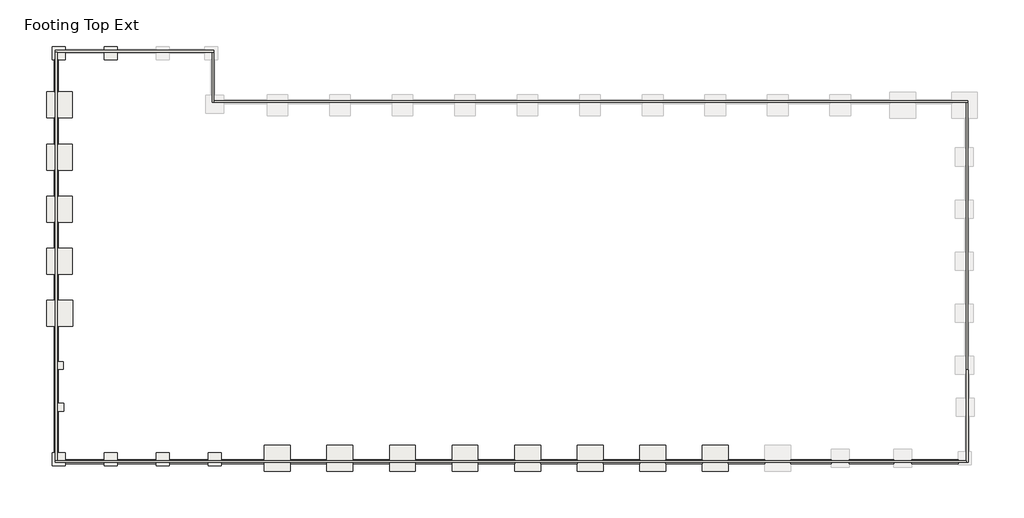
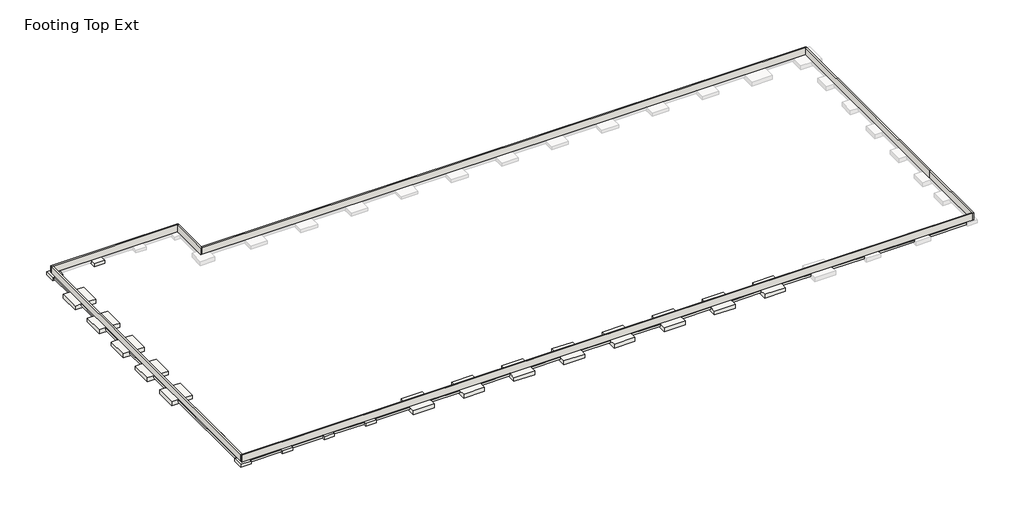
# One storey, part 1 of 2: 21 slabs, 7 walls, 2 footings.
"""IFC4 building model written with IfcOpenShell, lengths in millimetres."""

from ifc_helpers import new_model, si_unit, frame, origin, place, context, project, spatial, polyline, outline, extrude, faceted_brep, element, save

model = new_model("IFC4")

# Units and contexts
model_context = context("Model", 3, world=origin())
ifc_project = project(units=[si_unit("LENGTHUNIT", "METRE", prefix="MILLI")], contexts=[model_context])

# Site, building, storey
site = spatial("IfcSite", under=ifc_project)
building = spatial("IfcBuilding", under=site)
storey = spatial("IfcBuildingStorey", under=building, Name="Footing Top Ext", Elevation=-1066.8)

# Footings
placement = place(None, origin())
element("IfcFooting", 1, ObjectType="Bearing Footing - 18\" x 12\"", at=placement, inside=storey, context=model_context, shape_type="SweptSolid", body=[
    extrude(outline(polyline([(305655.7648264, -579216.5913841), (305655.7648264, -578759.3913841), (310230.9398264, -578759.3913841), (310230.9398264, -579216.5913841), (305655.7648264, -579216.5913841)])), frame((0.0, 0.0, -1371.6), z_axis=(0.0, 0.0, 1.0), x_axis=(1.0, 0.0, 0.0)), (0.0, 0.0, 1.0), 304.8),
    extrude(outline(polyline([(311754.9398264, -579216.5913841), (311754.9398264, -578759.3913841), (316361.8648264, -578759.3913841), (316361.8648264, -579216.5913841), (311754.9398264, -579216.5913841)])), frame((0.0, 0.0, -1371.6), z_axis=(0.0, 0.0, 1.0), x_axis=(1.0, 0.0, 0.0)), (0.0, 0.0, 1.0), 304.8),
    extrude(outline(polyline([(317885.8648264, -579216.5913841), (317885.8648264, -578759.3913841), (322457.8648264, -578759.3913841), (322457.8648264, -579216.5913841), (317885.8648264, -579216.5913841)])), frame((0.0, 0.0, -1371.6), z_axis=(0.0, 0.0, 1.0), x_axis=(1.0, 0.0, 0.0)), (0.0, 0.0, 1.0), 304.8),
    extrude(outline(polyline([(323981.8648264, -579216.5913841), (323981.8648264, -578759.3913841), (329077.7398264, -578759.3913841), (329077.7398264, -579216.5913841), (323981.8648264, -579216.5913841)])), frame((0.0, 0.0, -1371.6), z_axis=(0.0, 0.0, 1.0), x_axis=(1.0, 0.0, 0.0)), (0.0, 0.0, 1.0), 304.8),
    extrude(outline(polyline([(332125.7398264, -579216.5913841), (332125.7398264, -578759.3913841), (336431.0398264, -578759.3913841), (336431.0398264, -579216.5913841), (332125.7398264, -579216.5913841)])), frame((0.0, 0.0, -1371.6), z_axis=(0.0, 0.0, 1.0), x_axis=(1.0, 0.0, 0.0)), (0.0, 0.0, 1.0), 304.8),
    extrude(outline(polyline([(339479.0398264, -579216.5913841), (339479.0398264, -578759.3913841), (343784.3398264, -578759.3913841), (343784.3398264, -579216.5913841), (339479.0398264, -579216.5913841)])), frame((0.0, 0.0, -1371.6), z_axis=(0.0, 0.0, 1.0), x_axis=(1.0, 0.0, 0.0)), (0.0, 0.0, 1.0), 304.8),
    extrude(outline(polyline([(346832.3398264, -579216.5913841), (346832.3398264, -578759.3913841), (351137.6398264, -578759.3913841), (351137.6398264, -579216.5913841), (346832.3398264, -579216.5913841)])), frame((0.0, 0.0, -1371.6), z_axis=(0.0, 0.0, 1.0), x_axis=(1.0, 0.0, 0.0)), (0.0, 0.0, 1.0), 304.8),
    extrude(outline(polyline([(354185.6398264, -579216.5913841), (354185.6398264, -578759.3913841), (358490.9398264, -578759.3913841), (358490.9398264, -579216.5913841), (354185.6398264, -579216.5913841)])), frame((0.0, 0.0, -1371.6), z_axis=(0.0, 0.0, 1.0), x_axis=(1.0, 0.0, 0.0)), (0.0, 0.0, 1.0), 304.8),
    extrude(outline(polyline([(361538.9398264, -579216.5913841), (361538.9398264, -578759.3913841), (365844.2398264, -578759.3913841), (365844.2398264, -579216.5913841), (361538.9398264, -579216.5913841)])), frame((0.0, 0.0, -1371.6), z_axis=(0.0, 0.0, 1.0), x_axis=(1.0, 0.0, 0.0)), (0.0, 0.0, 1.0), 304.8),
    extrude(outline(polyline([(368892.2398264, -579216.5913841), (368892.2398264, -578759.3913841), (373197.5398264, -578759.3913841), (373197.5398264, -579216.5913841), (368892.2398264, -579216.5913841)])), frame((0.0, 0.0, -1371.6), z_axis=(0.0, 0.0, 1.0), x_axis=(1.0, 0.0, 0.0)), (0.0, 0.0, 1.0), 304.8),
    extrude(outline(polyline([(376245.5398264, -579216.5913841), (376245.5398264, -578759.3913841), (380550.8398264, -578759.3913841), (380550.8398264, -579216.5913841), (376245.5398264, -579216.5913841)])), frame((0.0, 0.0, -1371.6), z_axis=(0.0, 0.0, 1.0), x_axis=(1.0, 0.0, 0.0)), (0.0, 0.0, 1.0), 304.8),
    extrude(outline(polyline([(383598.8398264, -579216.5913841), (383598.8398264, -578759.3913841), (387904.1398264, -578759.3913841), (387904.1398264, -579216.5913841), (383598.8398264, -579216.5913841)])), frame((0.0, 0.0, -1371.6), z_axis=(0.0, 0.0, 1.0), x_axis=(1.0, 0.0, 0.0)), (0.0, 0.0, 1.0), 304.8),
    extrude(outline(polyline([(390952.1398264, -579216.5913841), (390952.1398264, -578759.3913841), (395714.6398264, -578759.3913841), (395714.6398264, -579216.5913841), (390952.1398264, -579216.5913841)])), frame((0.0, 0.0, -1371.6), z_axis=(0.0, 0.0, 1.0), x_axis=(1.0, 0.0, 0.0)), (0.0, 0.0, 1.0), 304.8),
    extrude(outline(polyline([(397848.2398264, -579216.5913841), (397848.2398264, -578759.3913841), (403067.9398264, -578759.3913841), (403067.9398264, -579216.5913841), (397848.2398264, -579216.5913841)])), frame((0.0, 0.0, -1371.6), z_axis=(0.0, 0.0, 1.0), x_axis=(1.0, 0.0, 0.0)), (0.0, 0.0, 1.0), 304.8),
    extrude(outline(polyline([(405201.5398264, -579216.5913841), (405201.5398264, -578759.3913841), (410675.2398264, -578759.3913841), (410675.2398264, -579216.5913841), (405201.5398264, -579216.5913841)])), frame((0.0, 0.0, -1371.6), z_axis=(0.0, 0.0, 1.0), x_axis=(1.0, 0.0, 0.0)), (0.0, 0.0, 1.0), 304.8),
])
element("IfcFooting", 2, ObjectType="Bearing Footing - 18\" x 12\"", at=placement, inside=storey, context=model_context, shape_type="SweptSolid", body=[
    extrude(outline(polyline([(304369.8898264, -531712.2413841), (304827.0898264, -531712.2413841), (304827.0898264, -535528.5913841), (304369.8898264, -535528.5913841), (304369.8898264, -531712.2413841)])), frame((0.0, 0.0, -1371.6), z_axis=(0.0, 0.0, 1.0), x_axis=(1.0, 0.0, 0.0)), (0.0, 0.0, 1.0), 304.8),
    extrude(outline(polyline([(304369.8898264, -538576.5913841), (304827.0898264, -538576.5913841), (304827.0898264, -541656.3413841), (304369.8898264, -541656.3413841), (304369.8898264, -538576.5913841)])), frame((0.0, 0.0, -1371.6), z_axis=(0.0, 0.0, 1.0), x_axis=(1.0, 0.0, 0.0)), (0.0, 0.0, 1.0), 304.8),
    extrude(outline(polyline([(304369.8898264, -544704.3413841), (304827.0898264, -544704.3413841), (304827.0898264, -547784.0913841), (304369.8898264, -547784.0913841), (304369.8898264, -544704.3413841)])), frame((0.0, 0.0, -1371.6), z_axis=(0.0, 0.0, 1.0), x_axis=(1.0, 0.0, 0.0)), (0.0, 0.0, 1.0), 304.8),
    extrude(outline(polyline([(304369.8898264, -550832.0913841), (304827.0898264, -550832.0913841), (304827.0898264, -553911.8413841), (304369.8898264, -553911.8413841), (304369.8898264, -550832.0913841)])), frame((0.0, 0.0, -1371.6), z_axis=(0.0, 0.0, 1.0), x_axis=(1.0, 0.0, 0.0)), (0.0, 0.0, 1.0), 304.8),
    extrude(outline(polyline([(304369.8898264, -556959.8413841), (304827.0898264, -556959.8413841), (304827.0898264, -560039.5913841), (304369.8898264, -560039.5913841), (304369.8898264, -556959.8413841)])), frame((0.0, 0.0, -1371.6), z_axis=(0.0, 0.0, 1.0), x_axis=(1.0, 0.0, 0.0)), (0.0, 0.0, 1.0), 304.8),
    extrude(outline(polyline([(304369.8898264, -563087.5913841), (304827.0898264, -563087.5913841), (304827.0898264, -567234.1413841), (304528.6398264, -567234.1413841), (304528.6398264, -568148.5413841), (304827.0898264, -568148.5413841), (304827.0898264, -572136.3413841), (304585.7898264, -572136.3413841), (304585.7898264, -573050.7413841), (304827.0898264, -573050.7413841), (304827.0898264, -577933.8913841), (304369.8898264, -577933.8913841), (304369.8898264, -563087.5913841)])), frame((0.0, 0.0, -1371.6), z_axis=(0.0, 0.0, 1.0), x_axis=(1.0, 0.0, 0.0)), (0.0, 0.0, 1.0), 304.8),
])

# Slabs
element("IfcSlab", 3, ObjectType="Footing-Rectangular : F10", at=placement, inside=storey, context=model_context, shape_type="Brep", body=[
    faceted_brep([(306509.8398264, -535528.5913841, -1066.8), (304827.0898264, -535528.5913841, -1066.8), (304369.8898264, -535528.5913841, -1066.8), (303461.8398264, -535528.5913841, -1066.8), (303461.8398264, -538576.5913841, -1066.8), (304369.8898264, -538576.5913841, -1066.8), (304827.0898264, -538576.5913841, -1066.8), (306509.8398264, -538576.5913841, -1066.8), (306509.8398264, -535528.5913841, -1676.4), (306509.8398264, -538576.5913841, -1676.4), (303461.8398264, -538576.5913841, -1676.4), (303461.8398264, -535528.5913841, -1676.4)], [[[0, 1, 2, 3, 4, 5, 6, 7]], [[8, 9, 10, 11]], [[3, 2, 1, 0, 8, 11]], [[4, 3, 11, 10]], [[7, 6, 5, 4, 10, 9]], [[0, 7, 9, 8]]]),
])
element("IfcSlab", 4, ObjectType="Footing-Rectangular : F10", at=placement, inside=storey, context=model_context, shape_type="Brep", body=[
    faceted_brep([(306509.8398264, -541656.3413841, -1066.8), (304827.0898264, -541656.3413841, -1066.8), (304369.8898264, -541656.3413841, -1066.8), (303461.8398264, -541656.3413841, -1066.8), (303461.8398264, -544704.3413841, -1066.8), (304369.8898264, -544704.3413841, -1066.8), (304827.0898264, -544704.3413841, -1066.8), (306509.8398264, -544704.3413841, -1066.8), (306509.8398264, -541656.3413841, -1676.4), (306509.8398264, -544704.3413841, -1676.4), (303461.8398264, -544704.3413841, -1676.4), (303461.8398264, -541656.3413841, -1676.4)], [[[0, 1, 2, 3, 4, 5, 6, 7]], [[8, 9, 10, 11]], [[3, 2, 1, 0, 8, 11]], [[4, 3, 11, 10]], [[7, 6, 5, 4, 10, 9]], [[0, 7, 9, 8]]]),
])
element("IfcSlab", 5, ObjectType="Footing-Rectangular : F10", at=placement, inside=storey, context=model_context, shape_type="Brep", body=[
    faceted_brep([(306509.8398264, -547784.0913841, -1066.8), (304827.0898264, -547784.0913841, -1066.8), (304369.8898264, -547784.0913841, -1066.8), (303461.8398264, -547784.0913841, -1066.8), (303461.8398264, -550832.0913841, -1066.8), (304369.8898264, -550832.0913841, -1066.8), (304827.0898264, -550832.0913841, -1066.8), (306509.8398264, -550832.0913841, -1066.8), (306509.8398264, -547784.0913841, -1676.4), (306509.8398264, -550832.0913841, -1676.4), (303461.8398264, -550832.0913841, -1676.4), (303461.8398264, -547784.0913841, -1676.4)], [[[0, 1, 2, 3, 4, 5, 6, 7]], [[8, 9, 10, 11]], [[3, 2, 1, 0, 8, 11]], [[4, 3, 11, 10]], [[7, 6, 5, 4, 10, 9]], [[0, 7, 9, 8]]]),
])
element("IfcSlab", 6, ObjectType="Footing-Rectangular : F10", at=placement, inside=storey, context=model_context, shape_type="Brep", body=[
    faceted_brep([(306509.8398264, -553911.8413841, -1066.8), (304827.0898264, -553911.8413841, -1066.8), (304369.8898264, -553911.8413841, -1066.8), (303461.8398264, -553911.8413841, -1066.8), (303461.8398264, -556959.8413841, -1066.8), (304369.8898264, -556959.8413841, -1066.8), (304827.0898264, -556959.8413841, -1066.8), (306509.8398264, -556959.8413841, -1066.8), (306509.8398264, -553911.8413841, -1676.4), (306509.8398264, -556959.8413841, -1676.4), (303461.8398264, -556959.8413841, -1676.4), (303461.8398264, -553911.8413841, -1676.4)], [[[0, 1, 2, 3, 4, 5, 6, 7]], [[8, 9, 10, 11]], [[3, 2, 1, 0, 8, 11]], [[4, 3, 11, 10]], [[7, 6, 5, 4, 10, 9]], [[0, 7, 9, 8]]]),
])
element("IfcSlab", 7, ObjectType="Footing-Rectangular : F10", at=placement, inside=storey, context=model_context, shape_type="Brep", body=[
    faceted_brep([(306516.1898264, -560039.5913841, -1066.8), (304827.0898264, -560039.5913841, -1066.8), (304369.8898264, -560039.5913841, -1066.8), (303468.1898264, -560039.5913841, -1066.8), (303468.1898264, -563087.5913841, -1066.8), (304369.8898264, -563087.5913841, -1066.8), (304827.0898264, -563087.5913841, -1066.8), (306516.1898264, -563087.5913841, -1066.8), (306516.1898264, -560039.5913841, -1676.4), (306516.1898264, -563087.5913841, -1676.4), (303468.1898264, -563087.5913841, -1676.4), (303468.1898264, -560039.5913841, -1676.4)], [[[0, 1, 2, 3, 4, 5, 6, 7]], [[8, 9, 10, 11]], [[3, 2, 1, 0, 8, 11]], [[4, 3, 11, 10]], [[7, 6, 5, 4, 10, 9]], [[0, 7, 9, 8]]]),
])
element("IfcSlab", 8, ObjectType="Footing-Rectangular : F10", at=placement, inside=storey, context=model_context, shape_type="Brep", body=[
    faceted_brep([(332125.7398264, -577079.8163841, -1066.8), (329077.7398264, -577079.8163841, -1066.8), (329077.7398264, -578759.3913841, -1066.8), (329077.7398264, -579216.5913841, -1066.8), (329077.7398264, -580127.8163841, -1066.8), (332125.7398264, -580127.8163841, -1066.8), (332125.7398264, -579216.5913841, -1066.8), (332125.7398264, -578759.3913841, -1066.8), (332125.7398264, -577079.8163841, -1676.4), (332125.7398264, -580127.8163841, -1676.4), (329077.7398264, -580127.8163841, -1676.4), (329077.7398264, -577079.8163841, -1676.4)], [[[0, 1, 2, 3, 4, 5, 6, 7]], [[8, 9, 10, 11]], [[1, 0, 8, 11]], [[4, 3, 2, 1, 11, 10]], [[5, 4, 10, 9]], [[0, 7, 6, 5, 9, 8]]]),
])
element("IfcSlab", 9, ObjectType="Footing-Rectangular : F10", at=placement, inside=storey, context=model_context, shape_type="Brep", body=[
    faceted_brep([(339479.0398264, -577079.8163841, -1066.8), (336431.0398264, -577079.8163841, -1066.8), (336431.0398264, -578759.3913841, -1066.8), (336431.0398264, -579216.5913841, -1066.8), (336431.0398264, -580127.8163841, -1066.8), (339479.0398264, -580127.8163841, -1066.8), (339479.0398264, -579216.5913841, -1066.8), (339479.0398264, -578759.3913841, -1066.8), (339479.0398264, -577079.8163841, -1676.4), (339479.0398264, -580127.8163841, -1676.4), (336431.0398264, -580127.8163841, -1676.4), (336431.0398264, -577079.8163841, -1676.4)], [[[0, 1, 2, 3, 4, 5, 6, 7]], [[8, 9, 10, 11]], [[1, 0, 8, 11]], [[4, 3, 2, 1, 11, 10]], [[5, 4, 10, 9]], [[0, 7, 6, 5, 9, 8]]]),
])
element("IfcSlab", 10, ObjectType="Footing-Rectangular : F10", at=placement, inside=storey, context=model_context, shape_type="Brep", body=[
    faceted_brep([(346832.3398264, -577079.8163841, -1066.8), (343784.3398264, -577079.8163841, -1066.8), (343784.3398264, -578759.3913841, -1066.8), (343784.3398264, -579216.5913841, -1066.8), (343784.3398264, -580127.8163841, -1066.8), (346832.3398264, -580127.8163841, -1066.8), (346832.3398264, -579216.5913841, -1066.8), (346832.3398264, -578759.3913841, -1066.8), (346832.3398264, -577079.8163841, -1676.4), (346832.3398264, -580127.8163841, -1676.4), (343784.3398264, -580127.8163841, -1676.4), (343784.3398264, -577079.8163841, -1676.4)], [[[0, 1, 2, 3, 4, 5, 6, 7]], [[8, 9, 10, 11]], [[1, 0, 8, 11]], [[4, 3, 2, 1, 11, 10]], [[5, 4, 10, 9]], [[0, 7, 6, 5, 9, 8]]]),
])
element("IfcSlab", 11, ObjectType="Footing-Rectangular : F10", at=placement, inside=storey, context=model_context, shape_type="Brep", body=[
    faceted_brep([(354185.6398264, -577079.8163841, -1066.8), (351137.6398264, -577079.8163841, -1066.8), (351137.6398264, -578759.3913841, -1066.8), (351137.6398264, -579216.5913841, -1066.8), (351137.6398264, -580127.8163841, -1066.8), (354185.6398264, -580127.8163841, -1066.8), (354185.6398264, -579216.5913841, -1066.8), (354185.6398264, -578759.3913841, -1066.8), (354185.6398264, -577079.8163841, -1676.4), (354185.6398264, -580127.8163841, -1676.4), (351137.6398264, -580127.8163841, -1676.4), (351137.6398264, -577079.8163841, -1676.4)], [[[0, 1, 2, 3, 4, 5, 6, 7]], [[8, 9, 10, 11]], [[1, 0, 8, 11]], [[4, 3, 2, 1, 11, 10]], [[5, 4, 10, 9]], [[0, 7, 6, 5, 9, 8]]]),
])
element("IfcSlab", 12, ObjectType="Footing-Rectangular : F10", at=placement, inside=storey, context=model_context, shape_type="Brep", body=[
    faceted_brep([(361538.9398264, -577079.8163841, -1066.8), (358490.9398264, -577079.8163841, -1066.8), (358490.9398264, -578759.3913841, -1066.8), (358490.9398264, -579216.5913841, -1066.8), (358490.9398264, -580127.8163841, -1066.8), (361538.9398264, -580127.8163841, -1066.8), (361538.9398264, -579216.5913841, -1066.8), (361538.9398264, -578759.3913841, -1066.8), (361538.9398264, -577079.8163841, -1676.4), (361538.9398264, -580127.8163841, -1676.4), (358490.9398264, -580127.8163841, -1676.4), (358490.9398264, -577079.8163841, -1676.4)], [[[0, 1, 2, 3, 4, 5, 6, 7]], [[8, 9, 10, 11]], [[1, 0, 8, 11]], [[4, 3, 2, 1, 11, 10]], [[5, 4, 10, 9]], [[0, 7, 6, 5, 9, 8]]]),
])
element("IfcSlab", 13, ObjectType="Footing-Rectangular : F10", at=placement, inside=storey, context=model_context, shape_type="Brep", body=[
    faceted_brep([(368892.2398264, -577079.8163841, -1066.8), (365844.2398264, -577079.8163841, -1066.8), (365844.2398264, -578759.3913841, -1066.8), (365844.2398264, -579216.5913841, -1066.8), (365844.2398264, -580127.8163841, -1066.8), (368892.2398264, -580127.8163841, -1066.8), (368892.2398264, -579216.5913841, -1066.8), (368892.2398264, -578759.3913841, -1066.8), (368892.2398264, -577079.8163841, -1676.4), (368892.2398264, -580127.8163841, -1676.4), (365844.2398264, -580127.8163841, -1676.4), (365844.2398264, -577079.8163841, -1676.4)], [[[0, 1, 2, 3, 4, 5, 6, 7]], [[8, 9, 10, 11]], [[1, 0, 8, 11]], [[4, 3, 2, 1, 11, 10]], [[5, 4, 10, 9]], [[0, 7, 6, 5, 9, 8]]]),
])
element("IfcSlab", 14, ObjectType="Footing-Rectangular : F10", at=placement, inside=storey, context=model_context, shape_type="Brep", body=[
    faceted_brep([(376245.5398264, -577079.8163841, -1066.8), (373197.5398264, -577079.8163841, -1066.8), (373197.5398264, -578759.3913841, -1066.8), (373197.5398264, -579216.5913841, -1066.8), (373197.5398264, -580127.8163841, -1066.8), (376245.5398264, -580127.8163841, -1066.8), (376245.5398264, -579216.5913841, -1066.8), (376245.5398264, -578759.3913841, -1066.8), (376245.5398264, -577079.8163841, -1676.4), (376245.5398264, -580127.8163841, -1676.4), (373197.5398264, -580127.8163841, -1676.4), (373197.5398264, -577079.8163841, -1676.4)], [[[0, 1, 2, 3, 4, 5, 6, 7]], [[8, 9, 10, 11]], [[1, 0, 8, 11]], [[4, 3, 2, 1, 11, 10]], [[5, 4, 10, 9]], [[0, 7, 6, 5, 9, 8]]]),
])
element("IfcSlab", 15, ObjectType="Footing-Rectangular : F10", at=placement, inside=storey, context=model_context, shape_type="Brep", body=[
    faceted_brep([(383598.8398264, -577079.8163841, -1066.8), (380550.8398264, -577079.8163841, -1066.8), (380550.8398264, -578759.3913841, -1066.8), (380550.8398264, -579216.5913841, -1066.8), (380550.8398264, -580127.8163841, -1066.8), (383598.8398264, -580127.8163841, -1066.8), (383598.8398264, -579216.5913841, -1066.8), (383598.8398264, -578759.3913841, -1066.8), (383598.8398264, -577079.8163841, -1676.4), (383598.8398264, -580127.8163841, -1676.4), (380550.8398264, -580127.8163841, -1676.4), (380550.8398264, -577079.8163841, -1676.4)], [[[0, 1, 2, 3, 4, 5, 6, 7]], [[8, 9, 10, 11]], [[1, 0, 8, 11]], [[4, 3, 2, 1, 11, 10]], [[5, 4, 10, 9]], [[0, 7, 6, 5, 9, 8]]]),
])
element("IfcSlab", 16, ObjectType="Footing-Rectangular : F5", at=placement, inside=storey, context=model_context, shape_type="Brep", body=[
    faceted_brep([(305655.7648264, -530188.2413841, -1066.8), (304131.7648264, -530188.2413841, -1066.8), (304131.7648264, -531712.2413841, -1066.8), (304369.8898264, -531712.2413841, -1066.8), (304827.0898264, -531712.2413841, -1066.8), (305655.7648264, -531712.2413841, -1066.8), (305655.7648264, -530975.6413841, -1066.8), (305655.7648264, -530518.4413841, -1066.8), (305655.7648264, -530188.2413841, -1524.0), (305655.7648264, -531712.2413841, -1524.0), (304131.7648264, -531712.2413841, -1524.0), (304131.7648264, -530188.2413841, -1524.0)], [[[0, 1, 2, 3, 4, 5, 6, 7]], [[8, 9, 10, 11]], [[1, 0, 8, 11]], [[2, 1, 11, 10]], [[5, 4, 3, 2, 10, 9]], [[0, 7, 6, 5, 9, 8]]]),
])
element("IfcSlab", 17, ObjectType="Footing-Rectangular : F5", at=placement, inside=storey, context=model_context, shape_type="Brep", body=[
    faceted_brep([(311754.9398264, -530191.4163841, -1066.8), (310230.9398264, -530191.4163841, -1066.8), (310230.9398264, -530518.4413841, -1066.8), (310230.9398264, -530975.6413841, -1066.8), (310230.9398264, -531715.4163841, -1066.8), (311754.9398264, -531715.4163841, -1066.8), (311754.9398264, -530975.6413841, -1066.8), (311754.9398264, -530518.4413841, -1066.8), (311754.9398264, -530191.4163841, -1524.0), (311754.9398264, -531715.4163841, -1524.0), (310230.9398264, -531715.4163841, -1524.0), (310230.9398264, -530191.4163841, -1524.0)], [[[0, 1, 2, 3, 4, 5, 6, 7]], [[8, 9, 10, 11]], [[1, 0, 8, 11]], [[4, 3, 2, 1, 11, 10]], [[5, 4, 10, 9]], [[0, 7, 6, 5, 9, 8]]]),
])
element("IfcSlab", 18, ObjectType="Footing-Rectangular : F5", at=placement, inside=storey, context=model_context, shape_type="Brep", body=[
    faceted_brep([(305655.7648264, -577933.8913841, -1066.8), (304827.0898264, -577933.8913841, -1066.8), (304369.8898264, -577933.8913841, -1066.8), (304131.7648264, -577933.8913841, -1066.8), (304131.7648264, -579457.8913841, -1066.8), (305655.7648264, -579457.8913841, -1066.8), (305655.7648264, -579216.5913841, -1066.8), (305655.7648264, -578759.3913841, -1066.8), (305655.7648264, -577933.8913841, -1524.0), (305655.7648264, -579457.8913841, -1524.0), (304131.7648264, -579457.8913841, -1524.0), (304131.7648264, -577933.8913841, -1524.0)], [[[0, 1, 2, 3, 4, 5, 6, 7]], [[8, 9, 10, 11]], [[3, 2, 1, 0, 8, 11]], [[4, 3, 11, 10]], [[5, 4, 10, 9]], [[0, 7, 6, 5, 9, 8]]]),
])
element("IfcSlab", 19, ObjectType="Footing-Rectangular : F5", at=placement, inside=storey, context=model_context, shape_type="Brep", body=[
    faceted_brep([(311754.9398264, -577930.7163841, -1066.8), (310230.9398264, -577930.7163841, -1066.8), (310230.9398264, -578759.3913841, -1066.8), (310230.9398264, -579216.5913841, -1066.8), (310230.9398264, -579454.7163841, -1066.8), (311754.9398264, -579454.7163841, -1066.8), (311754.9398264, -579216.5913841, -1066.8), (311754.9398264, -578759.3913841, -1066.8), (311754.9398264, -577930.7163841, -1524.0), (311754.9398264, -579454.7163841, -1524.0), (310230.9398264, -579454.7163841, -1524.0), (310230.9398264, -577930.7163841, -1524.0)], [[[0, 1, 2, 3, 4, 5, 6, 7]], [[8, 9, 10, 11]], [[1, 0, 8, 11]], [[4, 3, 2, 1, 11, 10]], [[5, 4, 10, 9]], [[0, 7, 6, 5, 9, 8]]]),
])
element("IfcSlab", 20, ObjectType="Footing-Rectangular : F5", at=placement, inside=storey, context=model_context, shape_type="Brep", body=[
    faceted_brep([(317885.8648264, -577930.7163841, -1066.8), (316361.8648264, -577930.7163841, -1066.8), (316361.8648264, -578759.3913841, -1066.8), (316361.8648264, -579216.5913841, -1066.8), (316361.8648264, -579454.7163841, -1066.8), (317885.8648264, -579454.7163841, -1066.8), (317885.8648264, -579216.5913841, -1066.8), (317885.8648264, -578759.3913841, -1066.8), (317885.8648264, -577930.7163841, -1524.0), (317885.8648264, -579454.7163841, -1524.0), (316361.8648264, -579454.7163841, -1524.0), (316361.8648264, -577930.7163841, -1524.0)], [[[0, 1, 2, 3, 4, 5, 6, 7]], [[8, 9, 10, 11]], [[1, 0, 8, 11]], [[4, 3, 2, 1, 11, 10]], [[5, 4, 10, 9]], [[0, 7, 6, 5, 9, 8]]]),
])
element("IfcSlab", 21, ObjectType="Footing-Rectangular : F5", at=placement, inside=storey, context=model_context, shape_type="Brep", body=[
    faceted_brep([(323981.8648264, -577933.8913841, -1066.8), (322457.8648264, -577933.8913841, -1066.8), (322457.8648264, -578759.3913841, -1066.8), (322457.8648264, -579216.5913841, -1066.8), (322457.8648264, -579457.8913841, -1066.8), (323981.8648264, -579457.8913841, -1066.8), (323981.8648264, -579216.5913841, -1066.8), (323981.8648264, -578759.3913841, -1066.8), (323981.8648264, -577933.8913841, -1524.0), (323981.8648264, -579457.8913841, -1524.0), (322457.8648264, -579457.8913841, -1524.0), (322457.8648264, -577933.8913841, -1524.0)], [[[0, 1, 2, 3, 4, 5, 6, 7]], [[8, 9, 10, 11]], [[1, 0, 8, 11]], [[4, 3, 2, 1, 11, 10]], [[5, 4, 10, 9]], [[0, 7, 6, 5, 9, 8]]]),
])
element("IfcSlab", 22, ObjectType="Footing-Rectangular : F6", at=placement, inside=storey, context=model_context, shape_type="Brep", body=[
    faceted_brep([(305443.0398264, -567234.1413841, -1066.8), (304827.0898264, -567234.1413841, -1066.8), (304528.6398264, -567234.1413841, -1066.8), (304528.6398264, -568148.5413841, -1066.8), (304827.0898264, -568148.5413841, -1066.8), (305443.0398264, -568148.5413841, -1066.8), (305443.0398264, -567234.1413841, -1371.6), (305443.0398264, -568148.5413841, -1371.6), (304827.0898264, -568148.5413841, -1371.6), (304528.6398264, -568148.5413841, -1371.6), (304528.6398264, -567234.1413841, -1371.6), (304827.0898264, -567234.1413841, -1371.6)], [[[0, 1, 2, 3, 4, 5]], [[6, 7, 8, 9, 10, 11]], [[2, 1, 0, 6, 11, 10]], [[3, 2, 10, 9]], [[5, 4, 3, 9, 8, 7]], [[0, 5, 7, 6]]]),
])
element("IfcSlab", 23, ObjectType="Footing-Rectangular : F6", at=placement, inside=storey, context=model_context, shape_type="Brep", body=[
    faceted_brep([(305500.1898264, -572136.3413841, -1066.8), (304827.0898264, -572136.3413841, -1066.8), (304585.7898264, -572136.3413841, -1066.8), (304585.7898264, -573050.7413841, -1066.8), (304827.0898264, -573050.7413841, -1066.8), (305500.1898264, -573050.7413841, -1066.8), (305500.1898264, -572136.3413841, -1371.6), (305500.1898264, -573050.7413841, -1371.6), (304827.0898264, -573050.7413841, -1371.6), (304585.7898264, -573050.7413841, -1371.6), (304585.7898264, -572136.3413841, -1371.6), (304827.0898264, -572136.3413841, -1371.6)], [[[0, 1, 2, 3, 4, 5]], [[6, 7, 8, 9, 10, 11]], [[2, 1, 0, 6, 11, 10]], [[3, 2, 10, 9]], [[5, 4, 3, 9, 8, 7]], [[0, 5, 7, 6]]]),
])

# Walls
element("IfcWall", 24, ObjectType="Frost Wall - 8\" Concrete", at=placement, inside=storey, context=model_context, shape_type="Brep", body=[
    faceted_brep([(304496.8898264, -530848.6413841, -1066.8), (304700.0898264, -530848.6413841, -1066.8), (322918.2398264, -530848.6413841, -1066.8), (323121.4398264, -530848.6413841, -1066.8), (323121.4398264, -530848.6413841, 0.0), (322918.2398264, -530848.6413841, 0.0), (304700.0898264, -530848.6413841, 0.0), (304496.8898264, -530848.6413841, 0.0), (304496.8898264, -530645.4413841, -1066.8), (304496.8898264, -530645.4413841, 0.0), (323121.4398264, -530645.4413841, 0.0), (323121.4398264, -530645.4413841, -1066.8)], [[[0, 1, 2, 3, 4, 5, 6, 7]], [[8, 9, 10, 11]], [[3, 2, 1, 0, 8, 11]], [[7, 6, 5, 4, 10, 9]], [[4, 3, 11, 10]], [[0, 7, 9, 8]]]),
])
element("IfcWall", 25, ObjectType="Frost Wall - 8\" Concrete", at=placement, inside=storey, context=model_context, shape_type="Brep", body=[
    faceted_brep([(322918.2398264, -530848.6413841, -1066.8), (322918.2398264, -536760.4913841, -1066.8), (322918.2398264, -536760.4913841, 0.0), (322918.2398264, -530848.6413841, 0.0), (323121.4398264, -530848.6413841, -1066.8), (323121.4398264, -530848.6413841, 0.0), (323121.4398264, -536557.2913841, 0.0), (323121.4398264, -536760.4913841, 0.0), (323121.4398264, -536760.4913841, -1066.8), (323121.4398264, -536557.2913841, -1066.8)], [[[0, 1, 2, 3]], [[4, 5, 6, 7, 8, 9]], [[1, 0, 4, 9, 8]], [[3, 2, 7, 6, 5]], [[0, 3, 5, 4]], [[2, 1, 8, 7]]]),
])
element("IfcWall", 26, ObjectType="Frost Wall - 8\" Concrete", at=placement, inside=storey, context=model_context, shape_type="Brep", body=[
    faceted_brep([(323121.4398264, -536760.4913841, -1066.8), (411564.2398264, -536760.4913841, -1066.8), (411767.4398264, -536760.4913841, -1066.8), (411767.4398264, -536760.4913841, 0.0), (411564.2398264, -536760.4913841, 0.0), (323121.4398264, -536760.4913841, 0.0), (323121.4398264, -536557.2913841, -1066.8), (323121.4398264, -536557.2913841, 0.0), (411767.4398264, -536557.2913841, 0.0), (411767.4398264, -536557.2913841, -1066.8)], [[[0, 1, 2, 3, 4, 5]], [[6, 7, 8, 9]], [[2, 1, 0, 6, 9]], [[5, 4, 3, 8, 7]], [[0, 5, 7, 6]], [[3, 2, 9, 8]]]),
])
element("IfcWall", 27, ObjectType="Frost Wall - 8\" Concrete", at=placement, inside=storey, context=model_context, shape_type="Brep", body=[
    faceted_brep([(411564.2398264, -536760.4913841, -1066.8), (411564.2398264, -568186.6413841, -1066.8), (411564.2398264, -568186.6413841, 0.0), (411564.2398264, -536760.4913841, 0.0), (411767.4398264, -536760.4913841, -1066.8), (411767.4398264, -536760.4913841, 0.0), (411767.4398264, -568186.6413841, 0.0), (411767.4398264, -568186.6413841, -1066.8), (411602.3398264, -568186.6413841, -1066.8), (411602.3398264, -568186.6413841, 0.0)], [[[0, 1, 2, 3]], [[4, 5, 6, 7]], [[1, 0, 4, 7, 8]], [[2, 1, 8, 7, 6, 9]], [[3, 2, 9, 6, 5]], [[0, 3, 5, 4]]]),
])
element("IfcWall", 28, ObjectType="Frost Wall - 8\" Concrete", at=placement, inside=storey, context=model_context, shape_type="Brep", body=[
    faceted_brep([(411602.3398264, -578886.3913841, -1066.8), (304700.0898264, -578886.3913841, -1066.8), (304496.8898264, -578886.3913841, -1066.8), (304496.8898264, -578886.3913841, 0.0), (304700.0898264, -578886.3913841, 0.0), (411602.3398264, -578886.3913841, 0.0), (411602.3398264, -579089.5913841, -1066.8), (411602.3398264, -579089.5913841, 0.0), (304496.8898264, -579089.5913841, 0.0), (304496.8898264, -579089.5913841, -1066.8)], [[[0, 1, 2, 3, 4, 5]], [[6, 7, 8, 9]], [[2, 1, 0, 6, 9]], [[5, 4, 3, 8, 7]], [[0, 5, 7, 6]], [[3, 2, 9, 8]]]),
])
element("IfcWall", 29, ObjectType="Frost Wall - 8\" Concrete", at=placement, inside=storey, context=model_context, shape_type="SweptSolid", body=[
    extrude(outline(polyline([(304700.0898264, -530848.6413841), (304700.0898264, -578886.3913841), (304496.8898264, -578886.3913841), (304496.8898264, -530848.6413841), (304700.0898264, -530848.6413841)])), frame((0.0, 0.0, -1066.8), z_axis=(0.0, 0.0, 1.0), x_axis=(1.0, 0.0, 0.0)), (0.0, 0.0, 1.0), 1066.8),
])
element("IfcWall", 30, ObjectType="Frost Wall - 8\" Concrete", at=placement, inside=storey, context=model_context, shape_type="Brep", body=[
    faceted_brep([(411602.3398264, -568186.6413841, -1066.8), (411602.3398264, -578886.3913841, -1066.8), (411602.3398264, -579089.5913841, -1066.8), (411602.3398264, -579089.5913841, 0.0), (411602.3398264, -578886.3913841, 0.0), (411602.3398264, -568186.6413841, 0.0), (411805.5398264, -568186.6413841, -1066.8), (411805.5398264, -568186.6413841, 0.0), (411805.5398264, -579089.5913841, 0.0), (411805.5398264, -579089.5913841, -1066.8), (411767.4398264, -568186.6413841, -1066.8), (411767.4398264, -568186.6413841, 0.0)], [[[0, 1, 2, 3, 4, 5]], [[6, 7, 8, 9]], [[2, 1, 0, 10, 6, 9]], [[5, 4, 3, 8, 7, 11]], [[0, 5, 11, 7, 6, 10]], [[3, 2, 9, 8]]]),
])

save(model, "model.ifc")

# Revit data of these elements
# Project information
#   Project Issue Date = "Issue Date"
#   Project Status = "Project Status"
#   Client Name = "Xcel"
#   Project Address = "Enter address here"
#   Project Name = "Sports Complex"
#   Project Number = "Project Number"
# Grids (mm)
#   "1-7": line (367368.24, -472874.843) -> (367368.24, -606417.413)
#   "1-6": line (374721.54, -472874.843) -> (374721.54, -606417.413)
#   "2-12": line (330601.74, -475922.843) -> (330601.74, -609465.413)
#   "1-12": line (330601.74, -472874.843) -> (330601.74, -606417.413)
#   "1-11": line (337955.04, -472874.843) -> (337955.04, -606417.413)
#   "1-10": line (345308.34, -472874.843) -> (345308.34, -606417.413)
#   "1-9": line (352661.64, -472874.843) -> (352661.64, -606417.413)
#   "1-8": line (360014.94, -472874.843) -> (360014.94, -606417.413)
#   "3-8": line (243887.399, -537052.591) -> (490605.763, -537052.591)
#   "3-3": line (243887.399, -567691.341) -> (490605.763, -567691.341)
#   "3-7": line (243887.399, -543180.341) -> (426856.7, -543180.341)
#   "3-6": line (243887.399, -549308.091) -> (426856.7, -549308.091)
#   "1-5": line (382074.84, -472874.843) -> (382074.84, -606417.413)
#   "1-4": line (389428.14, -472874.843) -> (389428.14, -606417.413)
#   "1-3": line (396781.44, -472874.843) -> (396781.44, -606417.413)
#   "1-2": line (404134.74, -472874.843) -> (404134.74, -606417.413)
#   "3-5": line (243887.399, -555435.841) -> (426856.7, -555435.841)
#   "3-4": line (243887.399, -561563.591) -> (426856.7, -561563.591)
#   "3-2": line (243887.399, -572593.541) -> (490605.763, -572593.541)
#   "3-B": line (310992.94, -472874.843) -> (310992.94, -606417.413)
#   "3-C": line (317120.69, -472874.843) -> (317120.69, -606417.413)
#   "3-1": line (243887.399, -578797.491) -> (490605.763, -578797.491)
#   "3-1.G": line (243887.399, -579000.691) -> (490605.763, -579000.691)
#   "3-E": line (323324.64, -472874.843) -> (323324.64, -606417.413)
#   "3-A": line (304788.99, -472803.223) -> (304788.99, -606345.792)
#   "3-A.G": line (304585.79, -472874.843) -> (304585.79, -606417.413)
#   "3-9": line (243887.399, -530848.641) -> (490605.763, -530848.641)
#   "3-9.G": line (243887.399, -530645.441) -> (490605.763, -530645.441)
#   "3-E.G": line (323527.84, -472874.843) -> (323527.84, -606417.413)
#   "3-3.G": line (243887.399, -567488.141) -> (490605.763, -567488.141)
#   "1-1G": line (411767.44, -472874.843) -> (411767.44, -606417.413)
#   "2-1": line (411564.24, -472874.843) -> (411564.24, -606417.413)
#   "1-1.G": line (411513.44, -472874.843) -> (411513.44, -606417.413)
#   "1-13": line (323121.44, -472874.843) -> (323121.44, -606417.413)
#   "1-A": line (243887.399, -567932.641) -> (426856.7, -567932.641)
#   "1-A.G": line (243887.399, -568186.641) -> (426856.7, -568186.641)
#   "1-13.G": line (322867.44, -472874.843) -> (322867.44, -606417.413)
#   "3-D": line (322918.24, -472874.843) -> (322918.24, -606417.413)
#   "1-F": line (243887.399, -536811.291) -> (426856.7, -536811.291)
#   "1-F.G": line (243887.399, -536557.291) -> (426856.7, -536557.291)
#   "3-D.G": line (323121.44, -472874.843) -> (323121.44, -606417.413)
#   "1-E": line (240890.199, -543180.341) -> (423859.5, -543180.341)
#   "1-D": line (240890.199, -549308.091) -> (423859.5, -549308.091)
#   "1-C": line (240890.199, -555435.841) -> (423859.5, -555435.841)
#   "1-B": line (240890.199, -561563.591) -> (423859.5, -561563.591)
#   "2-B": line (239924.999, -572593.541) -> (486643.363, -572593.541)
#   "2-A": line (240534.599, -578797.491) -> (487252.963, -578797.491)
#   "2-A.G": line (240534.599, -579000.691) -> (487252.963, -579000.691)
#   "2-7": line (367368.24, -475922.843) -> (367368.24, -609465.413)
#   "2-6": line (374721.54, -475922.843) -> (374721.54, -609465.413)
#   "2-5": line (382074.84, -475922.843) -> (382074.84, -609465.413)
#   "2-4": line (389428.14, -475922.843) -> (389428.14, -609465.413)
#   "2-3": line (396781.44, -475922.843) -> (396781.44, -609465.413)
#   "2-11": line (337955.04, -475922.843) -> (337955.04, -609465.413)
#   "2-10": line (345308.34, -475922.843) -> (345308.34, -609465.413)
#   "2-9": line (352661.64, -475922.843) -> (352661.64, -609465.413)
#   "2-8": line (360014.94, -475922.843) -> (360014.94, -609465.413)
#   "2-2": line (404134.74, -475922.843) -> (404134.74, -609465.413)
#   "2-13": line (323324.64, -475008.443) -> (323324.64, -608551.013)
#   "2-1G": line (411767.44, -476684.843) -> (411767.44, -610227.413)
#   "2-C": line (241753.799, -567932.641) -> (424723.1, -567932.641)
#   "2-3.G": line (396578.24, -475922.843) -> (396578.24, -609465.413)
# Type "Bearing Footing - 18\" x 12\""
#   Assembly Code = "A1010110"
# Type "Footing-Rectangular : F10"
#   Assembly Code = "A1010100"
#   Width = 10' - 0"
#   Length = 10' - 0"
#   Thickness = 2' - 0"
#   Structural Material [instance default] = Concrete, Cast-in-Place gray
# Type "Footing-Rectangular : F5"
#   Assembly Code = "A1010100"
#   Width = 5' - 0"
#   Length = 5' - 0"
#   Thickness = 1' - 6"
#   Structural Material [instance default] = Concrete, Cast-in-Place gray
# Type "Footing-Rectangular : F6"
#   Assembly Code = "A1010100"
#   Width = 3' - 0"
#   Length = 3' - 0"
#   Thickness = 1' - 0"
#   Structural Material [instance default] = Concrete, Cast-in-Place gray
# Type "Frost Wall - 8\" Concrete"
#   Assembly Code = "B2010"
#   Width = 0' - 8"
#   Layers, outside or top first: 0' - 8" "Concrete, Cast-in-Place gray" (function 1)
# Elements 1, 2 (IfcFooting, "Bearing Footing - 18\" x 12\"")
#   Phase Created = New Construction
#   Materials on its faces: "Concrete, Cast-in-Place gray"
# Elements 3, 4, 5, 6, 7, 8, 9, 10, 11, 12, 13, 14, 15 (IfcSlab, "Footing-Rectangular : F10")
#   Comments = ""
#   Structural Material = Concrete, Cast-in-Place gray
#   Phase Created = New Construction
#   Materials on its faces: "Concrete, Cast-in-Place gray"
# Elements 16, 17, 18, 19, 20, 21 (IfcSlab, "Footing-Rectangular : F5")
#   Comments = ""
#   Structural Material = Concrete, Cast-in-Place gray
#   Phase Created = New Construction
#   Materials on its faces: "Concrete, Cast-in-Place gray"
# Elements 22, 23 (IfcSlab, "Footing-Rectangular : F6")
#   Comments = ""
#   Structural Material = Concrete, Cast-in-Place gray
#   Phase Created = New Construction
#   Materials on its faces: "Concrete, Cast-in-Place gray"
# Elements 24, 25, 26, 27, 28, 29, 30 (IfcWall, "Frost Wall - 8\" Concrete")
#   Comments = ""
#   Top Offset = 0' - 0"
#   Base Offset = 0' - 0"
#   wall height = 3' - 6"
#   Phase Created = New Construction
#   Base Constraint = Footing Top Ext
#   Top Constraint = Level 1
#   Materials on its faces: "Concrete, Cast-in-Place gray"
# Materials
#   "Concrete, Cast-in-Place gray": class "Concrete", colour RGB 192 192 192, transparency 0, Description = "Cast-in-place concrete", Cost = 0
